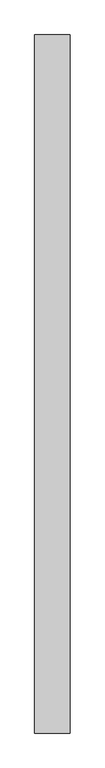
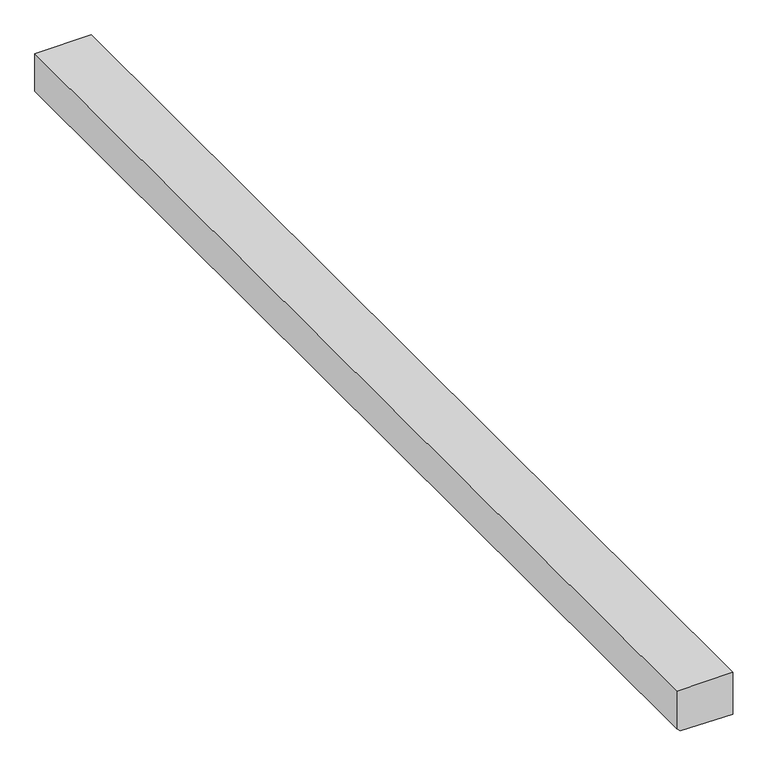
"""IFC4 building model written with IfcOpenShell, lengths in millimetres: proxy geometry, Blocking059 4:Blocking059 1918:306518 : Blocking059 4:Blocking059 1918:306518."""

from ifc_helpers import new_model, si_unit, frame, origin, place, context, project, spatial, polyline, outline, extrude, source, transform, mapped, element, save


def generic_models_c1256439(model_context):
    return source(origin(), model_context, "Body", "SweptSolid", [
        extrude(outline(polyline([(40038.291814, -2235.5979453), (40118.3092895, -2235.5979453), (40118.3092895, -2337.1979453), (40047.0174737, -2337.1979453), (40040.2769302, -2330.5659712), (40038.291814, -2235.5979453)])), frame((0.0, 7460.4857132, 0.0), z_axis=(0.0, 1.0, 0.0), x_axis=(0.0, 0.0, 1.0)), (0.0, 0.0, 1.0), 2000.0),
    ])


if __name__ == "__main__":
    model = new_model("IFC4")
    model_context = context("Model", 3, world=origin())
    ifc_project = project(units=[si_unit("LENGTHUNIT", "METRE", prefix="MILLI")], contexts=[model_context])
    site = spatial("IfcSite", under=ifc_project)
    building = spatial("IfcBuilding", under=site)
    placement = place(None, origin())
    generic_models_shape = generic_models_c1256439(model_context)
    element("IfcBuildingElementProxy", 1, Name="Blocking059 4:Blocking059 1918:306518 : Blocking059 4:Blocking059 1918:306518", ObjectType="Blocking059 4:Blocking059 1918:306518 : Blocking059 4:Blocking059 1918:306518", at=placement, inside=building, context=model_context, shape_type="MappedRepresentation", body=[
        mapped(generic_models_shape, transform((0.0, 0.0, 0.0), x_axis=(1.0, 0.0, 0.0), y_axis=(0.0, 1.0, 0.0), z_axis=(0.0, 0.0, 1.0))),
    ])
    save(model, "model.ifc")

# Revit data of these elements
# Type "Blocking059 4:Blocking059 1918:306518 : Blocking059 4:Blocking059 1918:306518"
#   NameOverride = "Blocking059 4:Blocking059 1918:306518"
#   ObjectTypeOverride = "Blocking059 4:Blocking059 1918"
#   Reference = "Blocking059 1918"
#   Category = "Generic Models"
#   Tag = "306518"
# Element 1 (IfcBuildingElementProxy, "Blocking059 4:Blocking059 1918:306518 : Blocking059 4:Blocking059 1918:306518")
#   Materials on its faces: "TREATED INTERMITTENT (FOR DRAINAGE) BLOCKING - SET IN BED OF SEALANT"
# Materials
#   "TREATED INTERMITTENT (FOR DRAINAGE) BLOCKING - SET IN BED OF SEALANT": class "Unassigned", colour RGB 140 161 107, transparency 0, Cost = 0
